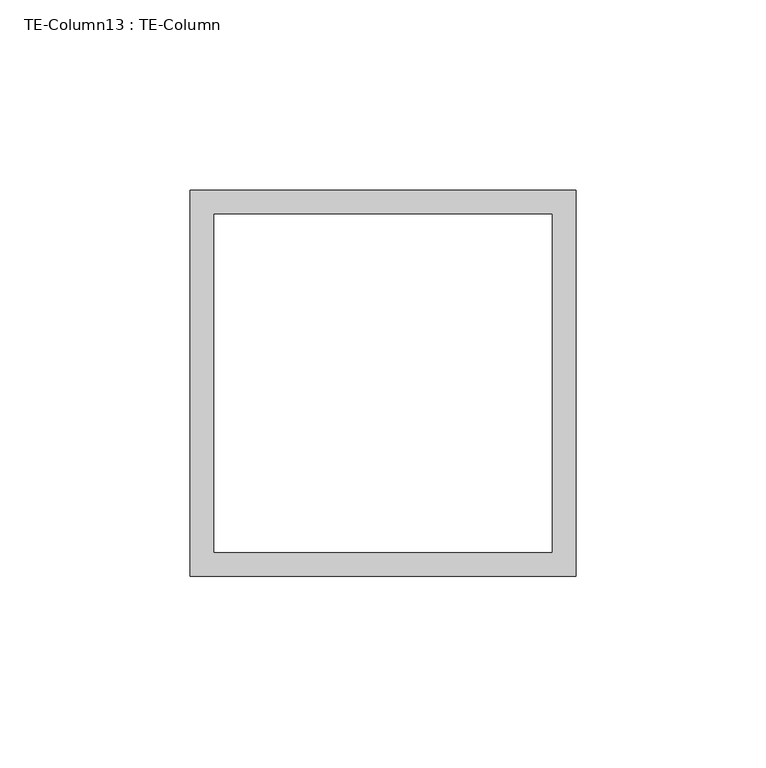
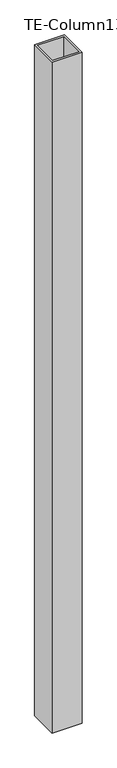
"""IFC4 building model written with IfcOpenShell, lengths in millimetres: proxy geometry, TE-Column13 : TE-Column."""

from ifc_helpers import new_model, si_unit, frame, origin, place, context, project, spatial, polyline, outline, extrude, source, transform, mapped, element, save


def te_column13_te_column_ebccfb0c(model_context):
    return source(origin(), model_context, "Body", "SweptSolid", [
        extrude(outline(polyline([(587468.2808739, -533991.8913841), (587468.2808739, -534093.4913841), (587366.6808739, -534093.4913841), (587366.6808739, -533991.8913841), (587468.2808739, -533991.8913841)]), holes=[polyline([(587373.0308739, -533998.2413841), (587373.0308739, -534087.1413841), (587461.9308739, -534087.1413841), (587461.9308739, -533998.2413841), (587373.0308739, -533998.2413841)])]), frame((0.0, 0.0, 28.575), z_axis=(0.0, 0.0, 1.0), x_axis=(1.0, 0.0, 0.0)), (0.0, 0.0, 1.0), 2406.65),
    ])


if __name__ == "__main__":
    model = new_model("IFC4")
    model_context = context("Model", 3, world=origin())
    ifc_project = project(units=[si_unit("LENGTHUNIT", "METRE", prefix="MILLI")], contexts=[model_context])
    site = spatial("IfcSite", under=ifc_project)
    building = spatial("IfcBuilding", under=site)
    placement = place(None, origin())
    te_column13_te_column_shape = te_column13_te_column_ebccfb0c(model_context)
    element("IfcBuildingElementProxy", 1, Name="TE-Column13 : TE-Column", ObjectType="TE-Column13 : TE-Column", at=placement, inside=building, context=model_context, shape_type="MappedRepresentation", body=[
        mapped(te_column13_te_column_shape, transform((0.0, 0.0, 0.0), x_axis=(1.0, 0.0, 0.0), y_axis=(0.0, 1.0, 0.0), z_axis=(0.0, 0.0, 1.0))),
    ])
    save(model, "model.ifc")

# Revit data of these elements
# Element 1 (IfcBuildingElementProxy, "TE-Column13 : TE-Column")
#   Materials on its faces: "4\"X4\" GALV. HSS TUBING"
# Materials
#   "4\"X4\" GALV. HSS TUBING": class "Generic", colour RGB 211 211 207, transparency 0, Cost = 0
